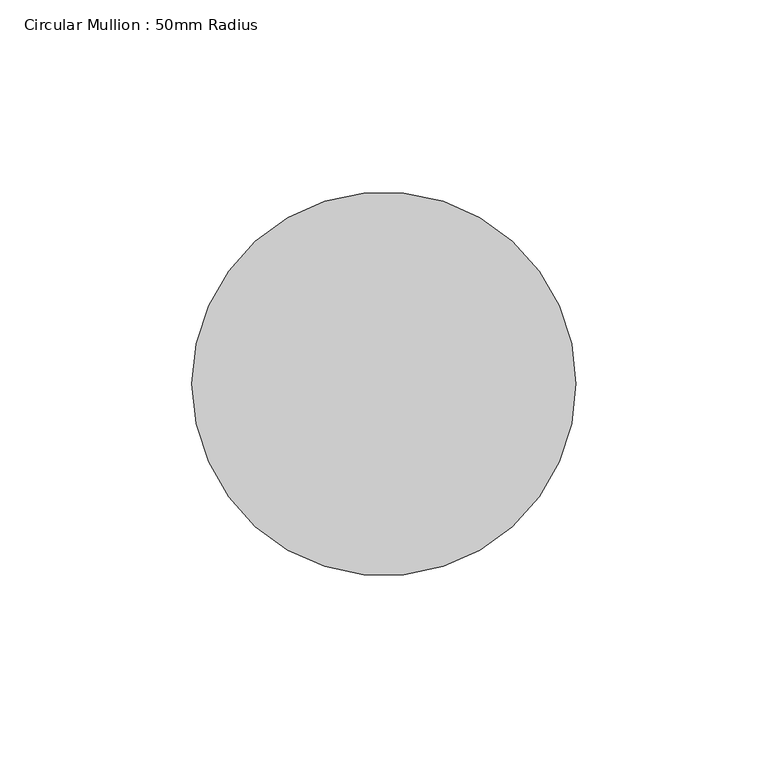
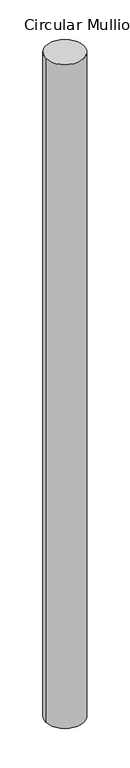
"""IFC4 building model written with IfcOpenShell, lengths in millimetres: member geometry, Circular Mullion : 50mm Radius."""

from ifc_helpers import new_model, si_unit, point, frame, frame_2d, origin, place, context, project, spatial, circle_curve, trimmed, segment, composite_curve, outline, extrude, source, transform, mapped, element, save


def circular_mullion_50mm_radius_8fa0eec3(model_context):
    return source(origin(), model_context, "Body", "SweptSolid", [
        extrude(outline(composite_curve([segment(trimmed(circle_curve(frame_2d((-50.0, 0.0)), 50.0), [point((0.0, 0.0))], [point((-100.0, 0.0))], False, "CARTESIAN"), True, "CONTINUOUS"), segment(trimmed(circle_curve(frame_2d((-50.0, 0.0)), 50.0), [point((-100.0, 0.0))], [point((0.0, 0.0))], False, "CARTESIAN"), True, "CONTINUOUS")], self_intersect=False)), frame((0.0, 0.0, -1850.0307572), z_axis=(0.0, 0.0, 1.0), x_axis=(1.0, 0.0, 0.0)), (0.0, 0.0, 1.0), 1850.0307572),
    ])


if __name__ == "__main__":
    model = new_model("IFC4")
    model_context = context("Model", 3, world=origin())
    ifc_project = project(units=[si_unit("LENGTHUNIT", "METRE", prefix="MILLI")], contexts=[model_context])
    site = spatial("IfcSite", under=ifc_project)
    building = spatial("IfcBuilding", under=site)
    placement = place(None, origin())
    circular_mullion_50mm_radius_shape = circular_mullion_50mm_radius_8fa0eec3(model_context)
    element("IfcMember", 1, ObjectType="Circular Mullion : 50mm Radius", at=placement, inside=building, context=model_context, shape_type="MappedRepresentation", body=[
        mapped(circular_mullion_50mm_radius_shape, transform((0.0, 0.0, 0.0), x_axis=(1.0, 0.0, 0.0), y_axis=(0.0, 1.0, 0.0), z_axis=(0.0, 0.0, 1.0))),
    ])
    save(model, "model.ifc")

# Revit data of these elements
# Type "Circular Mullion : 50mm Radius"
#   built-in parameter 1007350 = 0.164042 (stored number, unit not read)
# Element 1 (IfcMember, "Circular Mullion : 50mm Radius")
#   Materials on its faces: "Aluminium"
# Materials
#   "Aluminium": class "Metal", colour RGB 247 247 247, transparency 0, Description = "Aluminium 6061", Cost = 0
